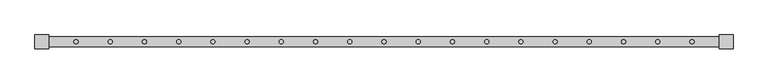
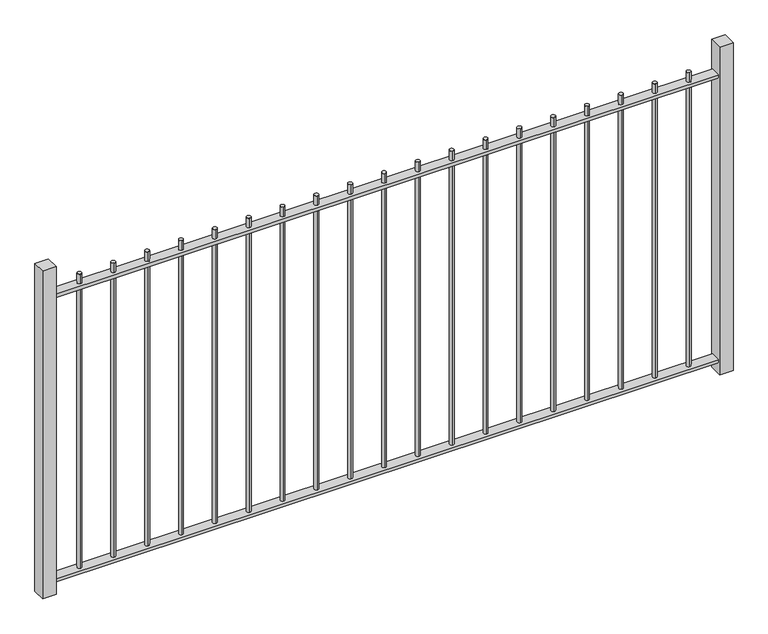
"""IFC4 building model written with IfcOpenShell, lengths in millimetres: railing geometry."""

from ifc_helpers import new_model, si_unit, point, frame, frame_2d, origin, place, context, project, spatial, polyline, circle_curve, trimmed, segment, composite_curve, outline, extrude, source, transform, mapped, element, save


def railing_aeaaafa9(model_context):
    return source(origin(), model_context, "Body", "SweptSolid", [
        extrude(outline(polyline([(-6519.419961, 92961.3203436), (-6519.419961, 93021.3203436), (-2519.419961, 93021.3203436), (-2519.419961, 92961.3203436), (-6519.419961, 92961.3203436)])), frame((0.0, 0.0, -30.0), z_axis=(0.0, 0.0, 1.0), x_axis=(1.0, 0.0, 0.0)), (0.0, 0.0, 1.0), 20.0),
        extrude(outline(polyline([(-6519.419961, 92961.3203436), (-6519.419961, 93021.3203436), (-2519.419961, 93021.3203436), (-2519.419961, 92961.3203436), (-6519.419961, 92961.3203436)])), frame((0.0, 0.0, 1750.0), z_axis=(0.0, 0.0, 1.0), x_axis=(1.0, 0.0, 0.0)), (0.0, 0.0, 1.0), 20.0),
        extrude(outline(composite_curve([segment(trimmed(circle_curve(frame_2d((-2719.419961, 92991.3203436)), 12.5), [point((-2719.419961, 92978.8203436))], [point((-2719.419961, 93003.8203436))], False, "CARTESIAN"), True, "CONTINUOUS"), segment(trimmed(circle_curve(frame_2d((-2719.419961, 92991.3203436)), 12.5), [point((-2719.419961, 93003.8203436))], [point((-2719.419961, 92978.8203436))], False, "CARTESIAN"), True, "CONTINUOUS")], self_intersect=False)), frame((0.0, 0.0, -10.0), z_axis=(0.0, 0.0, 1.0), x_axis=(1.0, 0.0, 0.0)), (0.0, 0.0, 1.0), 1840.0),
        extrude(outline(composite_curve([segment(trimmed(circle_curve(frame_2d((-2919.419961, 92991.3203436)), 12.5), [point((-2919.419961, 92978.8203436))], [point((-2919.419961, 93003.8203436))], False, "CARTESIAN"), True, "CONTINUOUS"), segment(trimmed(circle_curve(frame_2d((-2919.419961, 92991.3203436)), 12.5), [point((-2919.419961, 93003.8203436))], [point((-2919.419961, 92978.8203436))], False, "CARTESIAN"), True, "CONTINUOUS")], self_intersect=False)), frame((0.0, 0.0, -10.0), z_axis=(0.0, 0.0, 1.0), x_axis=(1.0, 0.0, 0.0)), (0.0, 0.0, 1.0), 1840.0),
        extrude(outline(composite_curve([segment(trimmed(circle_curve(frame_2d((-3119.419961, 92991.3203436)), 12.5), [point((-3119.419961, 92978.8203436))], [point((-3119.419961, 93003.8203436))], False, "CARTESIAN"), True, "CONTINUOUS"), segment(trimmed(circle_curve(frame_2d((-3119.419961, 92991.3203436)), 12.5), [point((-3119.419961, 93003.8203436))], [point((-3119.419961, 92978.8203436))], False, "CARTESIAN"), True, "CONTINUOUS")], self_intersect=False)), frame((0.0, 0.0, -10.0), z_axis=(0.0, 0.0, 1.0), x_axis=(1.0, 0.0, 0.0)), (0.0, 0.0, 1.0), 1840.0),
        extrude(outline(composite_curve([segment(trimmed(circle_curve(frame_2d((-3319.419961, 92991.3203436)), 12.5), [point((-3319.419961, 92978.8203436))], [point((-3319.419961, 93003.8203436))], False, "CARTESIAN"), True, "CONTINUOUS"), segment(trimmed(circle_curve(frame_2d((-3319.419961, 92991.3203436)), 12.5), [point((-3319.419961, 93003.8203436))], [point((-3319.419961, 92978.8203436))], False, "CARTESIAN"), True, "CONTINUOUS")], self_intersect=False)), frame((0.0, 0.0, -10.0), z_axis=(0.0, 0.0, 1.0), x_axis=(1.0, 0.0, 0.0)), (0.0, 0.0, 1.0), 1840.0),
        extrude(outline(composite_curve([segment(trimmed(circle_curve(frame_2d((-3519.419961, 92991.3203436)), 12.5), [point((-3519.419961, 92978.8203436))], [point((-3519.419961, 93003.8203436))], False, "CARTESIAN"), True, "CONTINUOUS"), segment(trimmed(circle_curve(frame_2d((-3519.419961, 92991.3203436)), 12.5), [point((-3519.419961, 93003.8203436))], [point((-3519.419961, 92978.8203436))], False, "CARTESIAN"), True, "CONTINUOUS")], self_intersect=False)), frame((0.0, 0.0, -10.0), z_axis=(0.0, 0.0, 1.0), x_axis=(1.0, 0.0, 0.0)), (0.0, 0.0, 1.0), 1840.0),
        extrude(outline(composite_curve([segment(trimmed(circle_curve(frame_2d((-3719.419961, 92991.3203436)), 12.5), [point((-3719.419961, 92978.8203436))], [point((-3719.419961, 93003.8203436))], False, "CARTESIAN"), True, "CONTINUOUS"), segment(trimmed(circle_curve(frame_2d((-3719.419961, 92991.3203436)), 12.5), [point((-3719.419961, 93003.8203436))], [point((-3719.419961, 92978.8203436))], False, "CARTESIAN"), True, "CONTINUOUS")], self_intersect=False)), frame((0.0, 0.0, -10.0), z_axis=(0.0, 0.0, 1.0), x_axis=(1.0, 0.0, 0.0)), (0.0, 0.0, 1.0), 1840.0),
        extrude(outline(composite_curve([segment(trimmed(circle_curve(frame_2d((-3919.419961, 92991.3203436)), 12.5), [point((-3919.419961, 92978.8203436))], [point((-3919.419961, 93003.8203436))], False, "CARTESIAN"), True, "CONTINUOUS"), segment(trimmed(circle_curve(frame_2d((-3919.419961, 92991.3203436)), 12.5), [point((-3919.419961, 93003.8203436))], [point((-3919.419961, 92978.8203436))], False, "CARTESIAN"), True, "CONTINUOUS")], self_intersect=False)), frame((0.0, 0.0, -10.0), z_axis=(0.0, 0.0, 1.0), x_axis=(1.0, 0.0, 0.0)), (0.0, 0.0, 1.0), 1840.0),
        extrude(outline(composite_curve([segment(trimmed(circle_curve(frame_2d((-4119.419961, 92991.3203436)), 12.5), [point((-4119.419961, 92978.8203436))], [point((-4119.419961, 93003.8203436))], False, "CARTESIAN"), True, "CONTINUOUS"), segment(trimmed(circle_curve(frame_2d((-4119.419961, 92991.3203436)), 12.5), [point((-4119.419961, 93003.8203436))], [point((-4119.419961, 92978.8203436))], False, "CARTESIAN"), True, "CONTINUOUS")], self_intersect=False)), frame((0.0, 0.0, -10.0), z_axis=(0.0, 0.0, 1.0), x_axis=(1.0, 0.0, 0.0)), (0.0, 0.0, 1.0), 1840.0),
        extrude(outline(composite_curve([segment(trimmed(circle_curve(frame_2d((-4319.419961, 92991.3203436)), 12.5), [point((-4319.419961, 92978.8203436))], [point((-4319.419961, 93003.8203436))], False, "CARTESIAN"), True, "CONTINUOUS"), segment(trimmed(circle_curve(frame_2d((-4319.419961, 92991.3203436)), 12.5), [point((-4319.419961, 93003.8203436))], [point((-4319.419961, 92978.8203436))], False, "CARTESIAN"), True, "CONTINUOUS")], self_intersect=False)), frame((0.0, 0.0, -10.0), z_axis=(0.0, 0.0, 1.0), x_axis=(1.0, 0.0, 0.0)), (0.0, 0.0, 1.0), 1840.0),
        extrude(outline(composite_curve([segment(trimmed(circle_curve(frame_2d((-4519.419961, 92991.3203436)), 12.5), [point((-4519.419961, 92978.8203436))], [point((-4519.419961, 93003.8203436))], False, "CARTESIAN"), True, "CONTINUOUS"), segment(trimmed(circle_curve(frame_2d((-4519.419961, 92991.3203436)), 12.5), [point((-4519.419961, 93003.8203436))], [point((-4519.419961, 92978.8203436))], False, "CARTESIAN"), True, "CONTINUOUS")], self_intersect=False)), frame((0.0, 0.0, -10.0), z_axis=(0.0, 0.0, 1.0), x_axis=(1.0, 0.0, 0.0)), (0.0, 0.0, 1.0), 1840.0),
        extrude(outline(composite_curve([segment(trimmed(circle_curve(frame_2d((-4719.419961, 92991.3203436)), 12.5), [point((-4719.419961, 92978.8203436))], [point((-4719.419961, 93003.8203436))], False, "CARTESIAN"), True, "CONTINUOUS"), segment(trimmed(circle_curve(frame_2d((-4719.419961, 92991.3203436)), 12.5), [point((-4719.419961, 93003.8203436))], [point((-4719.419961, 92978.8203436))], False, "CARTESIAN"), True, "CONTINUOUS")], self_intersect=False)), frame((0.0, 0.0, -10.0), z_axis=(0.0, 0.0, 1.0), x_axis=(1.0, 0.0, 0.0)), (0.0, 0.0, 1.0), 1840.0),
        extrude(outline(composite_curve([segment(trimmed(circle_curve(frame_2d((-4919.419961, 92991.3203436)), 12.5), [point((-4919.419961, 92978.8203436))], [point((-4919.419961, 93003.8203436))], False, "CARTESIAN"), True, "CONTINUOUS"), segment(trimmed(circle_curve(frame_2d((-4919.419961, 92991.3203436)), 12.5), [point((-4919.419961, 93003.8203436))], [point((-4919.419961, 92978.8203436))], False, "CARTESIAN"), True, "CONTINUOUS")], self_intersect=False)), frame((0.0, 0.0, -10.0), z_axis=(0.0, 0.0, 1.0), x_axis=(1.0, 0.0, 0.0)), (0.0, 0.0, 1.0), 1840.0),
        extrude(outline(composite_curve([segment(trimmed(circle_curve(frame_2d((-5119.419961, 92991.3203436)), 12.5), [point((-5119.419961, 92978.8203436))], [point((-5119.419961, 93003.8203436))], False, "CARTESIAN"), True, "CONTINUOUS"), segment(trimmed(circle_curve(frame_2d((-5119.419961, 92991.3203436)), 12.5), [point((-5119.419961, 93003.8203436))], [point((-5119.419961, 92978.8203436))], False, "CARTESIAN"), True, "CONTINUOUS")], self_intersect=False)), frame((0.0, 0.0, -10.0), z_axis=(0.0, 0.0, 1.0), x_axis=(1.0, 0.0, 0.0)), (0.0, 0.0, 1.0), 1840.0),
        extrude(outline(composite_curve([segment(trimmed(circle_curve(frame_2d((-5319.419961, 92991.3203436)), 12.5), [point((-5319.419961, 92978.8203436))], [point((-5319.419961, 93003.8203436))], False, "CARTESIAN"), True, "CONTINUOUS"), segment(trimmed(circle_curve(frame_2d((-5319.419961, 92991.3203436)), 12.5), [point((-5319.419961, 93003.8203436))], [point((-5319.419961, 92978.8203436))], False, "CARTESIAN"), True, "CONTINUOUS")], self_intersect=False)), frame((0.0, 0.0, -10.0), z_axis=(0.0, 0.0, 1.0), x_axis=(1.0, 0.0, 0.0)), (0.0, 0.0, 1.0), 1840.0),
        extrude(outline(composite_curve([segment(trimmed(circle_curve(frame_2d((-5519.419961, 92991.3203436)), 12.5), [point((-5519.419961, 92978.8203436))], [point((-5519.419961, 93003.8203436))], False, "CARTESIAN"), True, "CONTINUOUS"), segment(trimmed(circle_curve(frame_2d((-5519.419961, 92991.3203436)), 12.5), [point((-5519.419961, 93003.8203436))], [point((-5519.419961, 92978.8203436))], False, "CARTESIAN"), True, "CONTINUOUS")], self_intersect=False)), frame((0.0, 0.0, -10.0), z_axis=(0.0, 0.0, 1.0), x_axis=(1.0, 0.0, 0.0)), (0.0, 0.0, 1.0), 1840.0),
        extrude(outline(composite_curve([segment(trimmed(circle_curve(frame_2d((-5719.419961, 92991.3203436)), 12.5), [point((-5719.419961, 92978.8203436))], [point((-5719.419961, 93003.8203436))], False, "CARTESIAN"), True, "CONTINUOUS"), segment(trimmed(circle_curve(frame_2d((-5719.419961, 92991.3203436)), 12.5), [point((-5719.419961, 93003.8203436))], [point((-5719.419961, 92978.8203436))], False, "CARTESIAN"), True, "CONTINUOUS")], self_intersect=False)), frame((0.0, 0.0, -10.0), z_axis=(0.0, 0.0, 1.0), x_axis=(1.0, 0.0, 0.0)), (0.0, 0.0, 1.0), 1840.0),
        extrude(outline(composite_curve([segment(trimmed(circle_curve(frame_2d((-5919.419961, 92991.3203436)), 12.5), [point((-5919.419961, 92978.8203436))], [point((-5919.419961, 93003.8203436))], False, "CARTESIAN"), True, "CONTINUOUS"), segment(trimmed(circle_curve(frame_2d((-5919.419961, 92991.3203436)), 12.5), [point((-5919.419961, 93003.8203436))], [point((-5919.419961, 92978.8203436))], False, "CARTESIAN"), True, "CONTINUOUS")], self_intersect=False)), frame((0.0, 0.0, -10.0), z_axis=(0.0, 0.0, 1.0), x_axis=(1.0, 0.0, 0.0)), (0.0, 0.0, 1.0), 1840.0),
        extrude(outline(composite_curve([segment(trimmed(circle_curve(frame_2d((-6119.419961, 92991.3203436)), 12.5), [point((-6119.419961, 92978.8203436))], [point((-6119.419961, 93003.8203436))], False, "CARTESIAN"), True, "CONTINUOUS"), segment(trimmed(circle_curve(frame_2d((-6119.419961, 92991.3203436)), 12.5), [point((-6119.419961, 93003.8203436))], [point((-6119.419961, 92978.8203436))], False, "CARTESIAN"), True, "CONTINUOUS")], self_intersect=False)), frame((0.0, 0.0, -10.0), z_axis=(0.0, 0.0, 1.0), x_axis=(1.0, 0.0, 0.0)), (0.0, 0.0, 1.0), 1840.0),
        extrude(outline(composite_curve([segment(trimmed(circle_curve(frame_2d((-6319.419961, 92991.3203436)), 12.5), [point((-6319.419961, 92978.8203436))], [point((-6319.419961, 93003.8203436))], False, "CARTESIAN"), True, "CONTINUOUS"), segment(trimmed(circle_curve(frame_2d((-6319.419961, 92991.3203436)), 12.5), [point((-6319.419961, 93003.8203436))], [point((-6319.419961, 92978.8203436))], False, "CARTESIAN"), True, "CONTINUOUS")], self_intersect=False)), frame((0.0, 0.0, -10.0), z_axis=(0.0, 0.0, 1.0), x_axis=(1.0, 0.0, 0.0)), (0.0, 0.0, 1.0), 1840.0),
        extrude(outline(polyline([(-2559.419961, 93031.3203436), (-2479.419961, 93031.3203436), (-2479.419961, 92951.3203436), (-2559.419961, 92951.3203436), (-2559.419961, 93031.3203436)])), frame((0.0, 0.0, -100.0), z_axis=(0.0, 0.0, 1.0), x_axis=(1.0, 0.0, 0.0)), (0.0, 0.0, 1.0), 2050.0),
        extrude(outline(polyline([(-6559.419961, 93031.3203436), (-6479.419961, 93031.3203436), (-6479.419961, 92951.3203436), (-6559.419961, 92951.3203436), (-6559.419961, 93031.3203436)])), frame((0.0, 0.0, -100.0), z_axis=(0.0, 0.0, 1.0), x_axis=(1.0, 0.0, 0.0)), (0.0, 0.0, 1.0), 2050.0),
    ])


if __name__ == "__main__":
    model = new_model("IFC4")
    model_context = context("Model", 3, world=origin())
    ifc_project = project(units=[si_unit("LENGTHUNIT", "METRE", prefix="MILLI")], contexts=[model_context])
    site = spatial("IfcSite", under=ifc_project)
    building = spatial("IfcBuilding", under=site)
    placement = place(None, origin())
    railing_shape = railing_aeaaafa9(model_context)
    element("IfcRailing", 1, at=placement, inside=building, context=model_context, shape_type="MappedRepresentation", body=[
        mapped(railing_shape, transform((0.0, 0.0, 0.0), x_axis=(1.0, 0.0, 0.0), y_axis=(0.0, 1.0, 0.0), z_axis=(0.0, 0.0, 1.0))),
    ])
    save(model, "model.ifc")

# Revit data of these elements
# Element 1 (IfcRailing)
#   Materials on its faces: "NLRS_h2_staal_generiek zwart_gen_rsf", "NLRS_h2_staal_gen_rsf"
# Materials
#   "NLRS_h2_staal_generiek zwart_gen_rsf": class "Metal", colour RGB 189 187 185, transparency 0, Manufacturer = "RevitGG", URL = "www.revitgg.nl", Description = "Staal, generiek materiaal", Cost = 0
#   "NLRS_h2_staal_gen_rsf": class "H - Metaal", colour RGB 189 187 185, transparency 0, Keynote = "h2", Model = "generiek", Manufacturer = "Revit Standards Foundation", URL = "www.revitstandards.org", Description = "staal", Cost = 0
